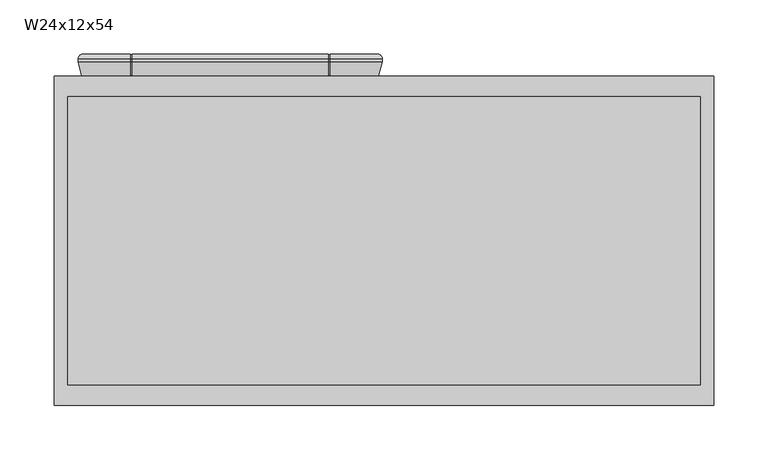
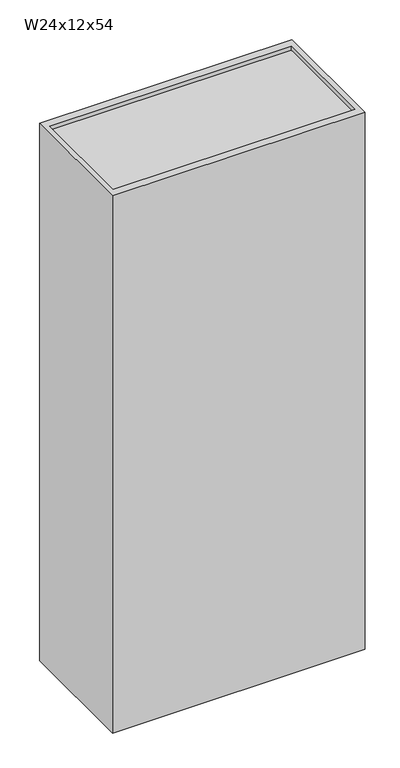
"""IFC4 building model written with IfcOpenShell, lengths in millimetres: furniture geometry, Cabinet-Wall-Merillat-Double_Door-Marlin : W24x12x54."""

from ifc_helpers import new_model, si_unit, frame, origin, place, context, project, spatial, polyline, circle_curve, ellipse_curve, outline, extrude, faceted_brep, source, transform, mapped, element, save
from ifc_brep_helpers import plane_surface, cylinder_surface, advanced_brep


def w24x12x54_3d81e8f6(model_context):
    return source(origin(), model_context, "Body", "SolidModel", [
        advanced_brep(
        [(-24.0971608, 382.5621, 2108.2), (-21.0006683, 387.0325, 2105.1035075), (-21.0006683, 387.0325, 790.4964925), (-24.0971608, 382.5621, 787.4), (-24.0971608, 379.7935, 787.4), (-24.0971608, 379.7935, 2108.2), (-20.5919608, 366.7125, 790.9052), (-20.5919608, 366.7125, 2104.6948), (24.104002, 366.7125, 2059.9988372), (24.104002, 366.7125, 835.6011628), (24.4741337, 367.50625, 835.9712945), (26.5552927, 371.96931, 838.0524535), (26.5552927, 371.96931, 2057.5475465), (24.4741337, 367.50625, 2059.6287055), (25.1555233, 374.2094093, 836.652684), (25.1555233, 374.2094093, 2058.947316), (10.8278392, 374.4595, 822.325), (10.8278392, 374.4595, 2073.275), (10.8278392, 379.2855, 822.325), (10.8278392, 379.2855, 2073.275), (25.1555233, 379.5355907, 836.652684), (25.1555233, 379.5355907, 2058.947316), (26.5552927, 381.77569, 838.0524535), (26.5552927, 381.77569, 2057.5475465), (24.4741337, 386.23875, 835.9712945), (24.1068694, 387.0263508, 835.6040302), (24.104002, 387.0325, 2059.9988372), (24.4741337, 386.23875, 2059.6287055), (24.1068694, 387.0325, 790.4964925), (24.1068694, 382.5621, 787.4), (253.7938467, 387.0325, 790.4964925), (256.8903392, 382.5621, 787.4), (208.7261206, 382.5621, 787.4), (208.7261206, 387.0325, 790.4964925), (25.6943694, 382.5621, 787.4), (25.6943694, 387.0325, 790.4964925), (207.1386206, 387.0325, 790.4964925), (207.1386206, 382.5621, 787.4), (24.1068694, 379.7935, 787.4), (256.8903392, 379.7935, 787.4), (208.7261206, 379.7935, 787.4), (25.6943694, 379.7935, 787.4), (207.1386206, 379.7935, 787.4), (24.1068694, 366.7125, 790.9052), (253.3851392, 366.7125, 790.9052), (208.7261206, 366.7125, 790.9052), (25.6943694, 366.7125, 790.9052), (207.1386206, 366.7125, 790.9052), (206.2378857, 371.96931, 838.0524535), (25.6943694, 367.50625, 835.9712945), (25.6943694, 366.7125, 835.6011628), (207.1386206, 366.7125, 835.6011628), (207.1386206, 367.50625, 835.9712945), (208.3190448, 367.50625, 835.9712945), (207.6376552, 374.2094093, 836.652684), (221.9653392, 374.4595, 822.325), (221.9653392, 379.2855, 822.325), (207.6376552, 379.5355907, 836.652684), (206.2378857, 381.77569, 838.0524535), (208.3190448, 386.23875, 835.9712945), (207.1386206, 386.23875, 835.9712945), (207.1386206, 387.0325, 835.6011628), (25.6943694, 387.0325, 835.6011628), (25.6943694, 386.23875, 835.9712945), (253.7938467, 387.0325, 2105.1035075), (256.8903392, 382.5621, 2108.2), (256.8903392, 379.7935, 2108.2), (253.3851392, 366.7125, 2104.6948), (208.6891765, 366.7125, 835.6011628), (208.6891765, 366.7125, 2059.9988372), (208.3190448, 367.50625, 2059.6287055), (206.2378857, 371.96931, 2057.5475465), (207.6376552, 374.2094093, 2058.947316), (221.9653392, 374.4595, 2073.275), (221.9653392, 379.2855, 2073.275), (207.6376552, 379.5355907, 2058.947316), (206.2378857, 381.77569, 2057.5475465), (208.3190448, 386.23875, 2059.6287055), (208.6891765, 387.0325, 2059.9988372), (208.6891765, 387.0325, 835.6011628), (208.7261206, 387.0325, 2105.1035075), (208.7261206, 382.5621, 2108.2), (24.1068694, 382.5621, 2108.2), (24.1068694, 387.0325, 2105.1035075), (207.1386206, 382.5621, 2108.2), (207.1386206, 387.0325, 2105.1035075), (25.6943694, 387.0325, 2105.1035075), (25.6943694, 382.5621, 2108.2), (208.7261206, 379.7935, 2108.2), (24.1068694, 379.7935, 2108.2), (207.1386206, 379.7935, 2108.2), (25.6943694, 379.7935, 2108.2), (208.7261206, 366.7125, 2104.6948), (24.1068694, 366.7125, 2104.6948), (207.1386206, 366.7125, 2104.6948), (25.6943694, 366.7125, 2104.6948), (207.1386206, 366.7125, 2059.9988372), (25.6943694, 366.7125, 2059.9988372), (207.1386206, 367.50625, 2059.6287055), (25.6943694, 367.50625, 2059.6287055), (25.6943694, 386.23875, 2059.6287055), (25.6943694, 387.0325, 2059.9988372), (207.1386206, 387.0325, 2059.9988372), (207.1386206, 386.23875, 2059.6287055), (207.1386206, 367.50625, 2104.0857412), (207.1386206, 379.8980037, 2107.40625), (207.1386206, 382.5621, 2107.40625), (207.1386206, 386.23875, 2104.9526052), (208.7261206, 386.23875, 2059.6287055), (208.7261206, 386.23875, 2104.9526052), (208.7261206, 382.5621, 2107.40625), (208.7261206, 379.8980037, 2107.40625), (208.7261206, 367.50625, 2104.0857412), (208.7261206, 367.50625, 2059.6287055), (24.1068694, 367.50625, 2059.6287055), (24.1068694, 367.50625, 2104.0857412), (24.1068694, 379.8980037, 2107.40625), (24.1068694, 382.5621, 2107.40625), (24.1068694, 386.23875, 2104.9526052), (24.1068694, 386.23875, 2059.6287055), (25.6943694, 386.23875, 2104.9526052), (25.6943694, 382.5621, 2107.40625), (25.6943694, 379.8980037, 2107.40625), (25.6943694, 367.50625, 2104.0857412), (24.1068694, 386.23875, 835.9712945), (24.1068694, 386.23875, 790.6473948), (24.1068694, 382.5621, 788.19375), (24.1068694, 379.8980037, 788.19375), (24.1068694, 367.50625, 791.5142588), (24.1068694, 367.50625, 835.9712945), (25.6943694, 367.50625, 791.5142588), (25.6943694, 379.8980037, 788.19375), (25.6943694, 382.5621, 788.19375), (25.6943694, 386.23875, 790.6473948), (207.1386206, 386.23875, 790.6473948), (207.1386206, 382.5621, 788.19375), (207.1386206, 379.8980037, 788.19375), (207.1386206, 367.50625, 791.5142588), (208.7261206, 386.23875, 835.9712945), (208.7261206, 367.50625, 835.9712945), (208.7261206, 367.50625, 791.5142588), (208.7261206, 379.8980037, 788.19375), (208.7261206, 382.5621, 788.19375), (208.7261206, 386.23875, 790.6473948)],
        [
            (0, 1, ellipse_curve(frame((-19.3219608, 382.5621, 2103.4248), z_axis=(-0.7071067811865475, 0.0, -0.7071067811865475), x_axis=(-0.7071067811865474, 0.0, 0.7071067811865476)), 6.7531526, 4.7752)),
            (1, 2),
            (2, 3, ellipse_curve(frame((-19.3219608, 382.5621, 792.1752), z_axis=(-0.7071067811865475, 0.0, 0.7071067811865475), x_axis=(0.7071067811865474, 0.0, 0.7071067811865476)), 6.7531526, 4.7752)),
            (3, 0),
            (3, 4),
            (4, 5),
            (5, 0),
            (4, 6),
            (6, 7),
            (7, 5),
            (8, 9),
            (9, 10),
            (10, 11),
            (11, 12),
            (12, 13),
            (13, 8),
            (11, 14, ellipse_curve(frame((25.1280392, 372.6348492, 836.6252), z_axis=(-0.7071067811865475, 0.0, 0.7071067811865475), x_axis=(0.7071067811865474, 0.0, 0.7071067811865476)), 2.2271035, 1.5748)),
            (14, 15),
            (15, 12, ellipse_curve(frame((25.1280392, 372.6348492, 2058.9748), z_axis=(-0.7071067811865475, 0.0, -0.7071067811865475), x_axis=(-0.7071067811865474, 0.0, 0.7071067811865476)), 2.2271035, 1.5748)),
            (14, 16),
            (16, 17),
            (17, 15),
            (16, 18),
            (18, 19),
            (19, 17),
            (18, 20),
            (20, 21),
            (21, 19),
            (20, 22, ellipse_curve(frame((25.1280392, 381.1101508, 836.6252), z_axis=(-0.7071067811865475, 0.0, 0.7071067811865475), x_axis=(0.7071067811865474, 0.0, 0.7071067811865476)), 2.2271035, 1.5748)),
            (22, 23),
            (23, 21, ellipse_curve(frame((25.1280392, 381.1101508, 2058.9748), z_axis=(-0.7071067811865475, 0.0, -0.7071067811865475), x_axis=(-0.7071067811865474, 0.0, 0.7071067811865476)), 2.2271035, 1.5748)),
            (22, 24),
            (24, 25),
            (25, 26),
            (26, 27),
            (27, 23),
            (2, 28),
            (28, 29, circle_curve(frame((24.1068694, 382.5621, 792.1752), z_axis=(-1.0, 0.0, 0.0), x_axis=(0.0, -1.0, 0.0)), 4.7752)),
            (29, 3),
            (30, 31, ellipse_curve(frame((252.1151392, 382.5621, 792.1752), z_axis=(-0.7071067811865475, 0.0, -0.7071067811865475), x_axis=(-0.7071067811865476, 0.0, 0.7071067811865474)), 6.7531526, 4.7752)),
            (31, 32),
            (32, 33, circle_curve(frame((208.7261206, 382.5621, 792.1752), z_axis=(1.0, 0.0, 0.0), x_axis=(0.0, -1.0, 0.0)), 4.7752)),
            (33, 30),
            (34, 35, circle_curve(frame((25.6943694, 382.5621, 792.1752), z_axis=(1.0, 0.0, 0.0), x_axis=(0.0, -1.0, 0.0)), 4.7752)),
            (35, 36),
            (36, 37, circle_curve(frame((207.1386206, 382.5621, 792.1752), z_axis=(-1.0, 0.0, 0.0), x_axis=(0.0, -1.0, 0.0)), 4.7752)),
            (37, 34),
            (29, 38),
            (38, 4),
            (31, 39),
            (39, 40),
            (40, 32),
            (41, 34),
            (37, 42),
            (42, 41),
            (38, 43),
            (43, 6),
            (39, 44),
            (44, 45),
            (45, 40),
            (46, 41),
            (42, 47),
            (47, 46),
            (48, 11),
            (10, 49),
            (49, 50),
            (50, 51),
            (51, 52),
            (52, 53),
            (53, 48),
            (48, 54, ellipse_curve(frame((207.6651392, 372.6348492, 836.6252), z_axis=(-0.7071067811865475, 0.0, -0.7071067811865475), x_axis=(-0.7071067811865476, 0.0, 0.7071067811865474)), 2.2271035, 1.5748)),
            (54, 14),
            (54, 55),
            (55, 16),
            (55, 56),
            (56, 18),
            (56, 57),
            (57, 20),
            (57, 58, ellipse_curve(frame((207.6651392, 381.1101508, 836.6252), z_axis=(-0.7071067811865475, 0.0, -0.7071067811865475), x_axis=(-0.7071067811865476, 0.0, 0.7071067811865474)), 2.2271035, 1.5748)),
            (58, 22),
            (58, 59),
            (59, 60),
            (60, 61),
            (61, 62),
            (62, 63),
            (63, 24),
            (30, 64),
            (64, 65, ellipse_curve(frame((252.1151392, 382.5621, 2103.4248), z_axis=(0.7071067811865475, 0.0, -0.7071067811865475), x_axis=(-0.7071067811865474, 0.0, -0.7071067811865476)), 6.7531526, 4.7752)),
            (65, 31),
            (65, 66),
            (66, 39),
            (66, 67),
            (67, 44),
            (68, 69),
            (69, 70),
            (70, 71),
            (71, 48),
            (53, 68),
            (71, 72, ellipse_curve(frame((207.6651392, 372.6348492, 2058.9748), z_axis=(0.7071067811865475, 0.0, -0.7071067811865475), x_axis=(-0.7071067811865474, 0.0, -0.7071067811865476)), 2.2271035, 1.5748)),
            (72, 54),
            (72, 73),
            (73, 55),
            (73, 74),
            (74, 56),
            (74, 75),
            (75, 57),
            (75, 76, ellipse_curve(frame((207.6651392, 381.1101508, 2058.9748), z_axis=(0.7071067811865475, 0.0, -0.7071067811865475), x_axis=(-0.7071067811865474, 0.0, -0.7071067811865476)), 2.2271035, 1.5748)),
            (76, 58),
            (76, 77),
            (77, 78),
            (78, 79),
            (79, 59),
            (64, 80),
            (80, 81, circle_curve(frame((208.7261206, 382.5621, 2103.4248), z_axis=(1.0, 0.0, 0.0), x_axis=(0.0, -1.0, 0.0)), 4.7752)),
            (81, 65),
            (0, 82),
            (82, 83, circle_curve(frame((24.1068694, 382.5621, 2103.4248), z_axis=(-1.0, 0.0, 0.0), x_axis=(0.0, -1.0, 0.0)), 4.7752)),
            (83, 1),
            (84, 85, circle_curve(frame((207.1386206, 382.5621, 2103.4248), z_axis=(-1.0, 0.0, 0.0), x_axis=(0.0, -1.0, 0.0)), 4.7752)),
            (85, 86),
            (86, 87, circle_curve(frame((25.6943694, 382.5621, 2103.4248), z_axis=(1.0, 0.0, 0.0), x_axis=(0.0, -1.0, 0.0)), 4.7752)),
            (87, 84),
            (81, 88),
            (88, 66),
            (5, 89),
            (89, 82),
            (90, 84),
            (87, 91),
            (91, 90),
            (88, 92),
            (92, 67),
            (7, 93),
            (93, 89),
            (94, 90),
            (91, 95),
            (95, 94),
            (43, 9),
            (8, 93),
            (92, 69),
            (68, 45),
            (96, 94),
            (95, 97),
            (97, 96),
            (50, 46),
            (47, 51),
            (12, 71),
            (70, 98),
            (98, 96),
            (97, 99),
            (99, 13),
            (15, 72),
            (17, 73),
            (19, 74),
            (21, 75),
            (23, 76),
            (27, 100),
            (100, 101),
            (101, 102),
            (102, 103),
            (103, 77),
            (83, 26),
            (25, 28),
            (33, 79),
            (78, 80),
            (85, 102),
            (101, 86),
            (35, 62),
            (61, 36),
            (98, 104),
            (104, 105),
            (105, 106),
            (106, 107, circle_curve(frame((207.1386206, 382.5621, 2103.4248), z_axis=(-1.0, 0.0, 0.0), x_axis=(0.0, 0.0, 1.0)), 3.98145)),
            (107, 103),
            (78, 108),
            (108, 109),
            (109, 110, circle_curve(frame((208.7261206, 382.5621, 2103.4248), z_axis=(1.0, 0.0, 0.0), x_axis=(0.0, 0.0, 1.0)), 3.98145)),
            (110, 111),
            (111, 112),
            (112, 113),
            (113, 69),
            (77, 108),
            (107, 109),
            (106, 110),
            (105, 111),
            (104, 112),
            (70, 113),
            (8, 114),
            (114, 115),
            (115, 116),
            (116, 117),
            (117, 118, circle_curve(frame((24.1068694, 382.5621, 2103.4248), z_axis=(-1.0, 0.0, 0.0), x_axis=(0.0, 0.0, 1.0)), 3.98145)),
            (118, 119),
            (119, 26),
            (100, 120),
            (120, 121, circle_curve(frame((25.6943694, 382.5621, 2103.4248), z_axis=(1.0, 0.0, 0.0), x_axis=(0.0, 0.0, 1.0)), 3.98145)),
            (121, 122),
            (122, 123),
            (123, 99),
            (119, 27),
            (118, 120),
            (117, 121),
            (116, 122),
            (115, 123),
            (114, 13),
            (25, 124),
            (124, 125),
            (125, 126, circle_curve(frame((24.1068694, 382.5621, 792.1752), z_axis=(-1.0, 0.0, 0.0), x_axis=(0.0, 0.0, 1.0)), 3.98145)),
            (126, 127),
            (127, 128),
            (128, 129),
            (129, 9),
            (49, 130),
            (130, 131),
            (131, 132),
            (132, 133, circle_curve(frame((25.6943694, 382.5621, 792.1752), z_axis=(1.0, 0.0, 0.0), x_axis=(0.0, 0.0, 1.0)), 3.98145)),
            (133, 63),
            (129, 10),
            (128, 130),
            (127, 131),
            (126, 132),
            (125, 133),
            (124, 24),
            (60, 134),
            (134, 135, circle_curve(frame((207.1386206, 382.5621, 792.1752), z_axis=(-1.0, 0.0, 0.0), x_axis=(0.0, 0.0, 1.0)), 3.98145)),
            (135, 136),
            (136, 137),
            (137, 52),
            (138, 79),
            (68, 139),
            (139, 140),
            (140, 141),
            (141, 142),
            (142, 143, circle_curve(frame((208.7261206, 382.5621, 792.1752), z_axis=(1.0, 0.0, 0.0), x_axis=(0.0, 0.0, 1.0)), 3.98145)),
            (143, 138),
            (138, 59),
            (53, 139),
            (137, 140),
            (136, 141),
            (135, 142),
            (134, 143),
        ],
        [
            cylinder_surface(frame((-19.3219608, 382.5621, 2108.2), z_axis=(0.0, 0.0, 1.0), x_axis=(0.0, -1.0, 0.0)), 4.7752),
            plane_surface(frame((-24.0971608, 382.5621, 2108.2), z_axis=(-1.0, 0.0, 0.0), x_axis=(0.0, 0.0, -1.0))),
            plane_surface(frame((-24.0971608, 379.7935, 2108.2), z_axis=(-0.9659229350723619, -0.25882983502910506, 0.0), x_axis=(0.0, 0.0, -1.0))),
            plane_surface(frame((24.104002, 366.7125, 2059.9988372), z_axis=(0.9063077870366099, -0.4226182617407856, 0.0), x_axis=(0.0, 0.0, -1.0))),
            cylinder_surface(frame((25.1280392, 372.6348492, 2108.2), z_axis=(0.0, 0.0, 1.0000000000000002), x_axis=(0.01745240643729364, 0.9998476951563912, 0.0)), 1.5748),
            plane_surface(frame((25.1555233, 374.2094093, 2058.947316), z_axis=(0.017452406437322144, 0.9998476951563906, 0.0), x_axis=(0.0, 0.0, -1.0))),
            plane_surface(frame((10.8278392, 374.4595, 2073.275), z_axis=(1.0, 0.0, 0.0), x_axis=(0.0, 0.0, -1.0))),
            plane_surface(frame((10.8278392, 379.2855, 2073.275), z_axis=(0.01745240643727848, -0.9998476951563914, 0.0), x_axis=(0.0, 0.0, -1.0))),
            cylinder_surface(frame((25.1280392, 381.1101508, 2108.2), z_axis=(0.0, 0.0, 1.0000000000000002), x_axis=(0.9063077870367326, 0.42261826174052236, 0.0)), 1.5748),
            plane_surface(frame((26.5552927, 381.77569, 2057.5475465), z_axis=(0.9063077870366333, 0.4226182617407352, 0.0), x_axis=(0.0, 0.0, -1.0))),
            cylinder_surface(frame((-24.0971608, 382.5621, 792.1752), z_axis=(-1.0, 0.0, 0.0), x_axis=(0.0, -1.0, 0.0)), 4.7752),
            plane_surface(frame((-24.0971608, 382.5621, 787.4), z_axis=(0.0, 0.0, -1.0), x_axis=(1.0, 0.0, 0.0))),
            plane_surface(frame((-24.0971608, 379.7935, 787.4), z_axis=(0.0, -0.2588298350291095, -0.9659229350723607), x_axis=(1.0, 0.0, 0.0))),
            plane_surface(frame((24.104002, 366.7125, 835.6011628), z_axis=(0.0, -0.42261826174078143, 0.9063077870366119), x_axis=(1.0, 0.0, 0.0))),
            cylinder_surface(frame((-24.0971608, 372.6348492, 836.6252), z_axis=(-1.0000000000000002, 0.0, 0.0), x_axis=(0.0, 0.9998476951563913, 0.017452406437289025)), 1.5748),
            plane_surface(frame((25.1555233, 374.2094093, 836.652684), z_axis=(0.0, 0.9998476951563907, 0.01745240643731753), x_axis=(1.0, 0.0, 0.0))),
            plane_surface(frame((10.8278392, 374.4595, 822.325), z_axis=(0.0, 0.0, 1.0), x_axis=(1.0, 0.0, 0.0))),
            plane_surface(frame((10.8278392, 379.2855, 822.325), z_axis=(0.0, -0.9998476951563913, 0.017452406437283095), x_axis=(1.0, 0.0, 0.0))),
            cylinder_surface(frame((-24.0971608, 381.1101508, 836.6252), z_axis=(-1.0000000000000002, 0.0, 0.0), x_axis=(0.0, 0.4226182617405265, 0.9063077870367306)), 1.5748),
            plane_surface(frame((26.5552927, 381.77569, 838.0524535), z_axis=(0.0, 0.4226182617407394, 0.9063077870366314), x_axis=(1.0, 0.0, 0.0))),
            cylinder_surface(frame((252.1151392, 382.5621, 787.4), z_axis=(0.0, 0.0, -1.0), x_axis=(0.0, -1.0, 0.0)), 4.7752),
            plane_surface(frame((256.8903392, 382.5621, 787.4), z_axis=(1.0, 0.0, 0.0), x_axis=(0.0, 0.0, 1.0))),
            plane_surface(frame((256.8903392, 379.7935, 787.4), z_axis=(0.9659229350723619, -0.25882983502910506, 0.0), x_axis=(0.0, 0.0, 1.0))),
            plane_surface(frame((208.6891765, 366.7125, 835.6011628), z_axis=(-0.9063077870366099, -0.4226182617407856, 0.0), x_axis=(0.0, 0.0, 1.0))),
            cylinder_surface(frame((207.6651392, 372.6348492, 787.4), z_axis=(0.0, 0.0, -1.0000000000000002), x_axis=(-0.01745240643729364, 0.9998476951563912, 0.0)), 1.5748),
            plane_surface(frame((207.6376552, 374.2094093, 836.652684), z_axis=(-0.017452406437322144, 0.9998476951563906, 0.0), x_axis=(0.0, 0.0, 1.0))),
            plane_surface(frame((221.9653392, 374.4595, 822.325), z_axis=(-1.0, 0.0, 0.0), x_axis=(0.0, 0.0, 1.0))),
            plane_surface(frame((221.9653392, 379.2855, 822.325), z_axis=(-0.01745240643727848, -0.9998476951563914, 0.0), x_axis=(0.0, 0.0, 1.0))),
            cylinder_surface(frame((207.6651392, 381.1101508, 787.4), z_axis=(0.0, 0.0, -1.0000000000000002), x_axis=(-0.9063077870367326, 0.42261826174052236, 0.0)), 1.5748),
            plane_surface(frame((206.2378857, 381.77569, 838.0524535), z_axis=(-0.9063077870366333, 0.4226182617407352, 0.0), x_axis=(0.0, 0.0, 1.0))),
            cylinder_surface(frame((256.8903392, 382.5621, 2103.4248), z_axis=(1.0, 0.0, 0.0), x_axis=(0.0, -1.0, 0.0)), 4.7752),
            plane_surface(frame((256.8903392, 382.5621, 2108.2), z_axis=(0.0, 0.0, 1.0), x_axis=(-1.0, 0.0, 0.0))),
            plane_surface(frame((256.8903392, 379.7935, 2108.2), z_axis=(0.0, -0.2588298350291006, 0.9659229350723632), x_axis=(-1.0, 0.0, 0.0))),
            plane_surface(frame((253.3851392, 366.7125, 2104.6948), z_axis=(0.0, -1.0, 0.0), x_axis=(-1.0, 0.0, 0.0))),
            plane_surface(frame((208.6891765, 366.7125, 2059.9988372), z_axis=(0.0, -0.42261826174078976, -0.9063077870366079), x_axis=(-1.0, 0.0, 0.0))),
            cylinder_surface(frame((256.8903392, 372.6348492, 2058.9748), z_axis=(1.0000000000000002, 0.0, 0.0), x_axis=(0.0, 0.999847695156391, -0.017452406437298253)), 1.5748),
            plane_surface(frame((207.6376552, 374.2094093, 2058.947316), z_axis=(0.0, 0.9998476951563905, -0.01745240643732676), x_axis=(-1.0, 0.0, 0.0))),
            plane_surface(frame((221.9653392, 374.4595, 2073.275), z_axis=(0.0, 0.0, -1.0), x_axis=(-1.0, 0.0, 0.0))),
            plane_surface(frame((221.9653392, 379.2855, 2073.275), z_axis=(0.0, -0.9998476951563915, -0.017452406437273867), x_axis=(-1.0, 0.0, 0.0))),
            cylinder_surface(frame((256.8903392, 381.1101508, 2058.9748), z_axis=(1.0000000000000002, 0.0, 0.0), x_axis=(0.0, 0.4226182617405182, -0.9063077870367346)), 1.5748),
            plane_surface(frame((206.2378857, 381.77569, 2057.5475465), z_axis=(0.0, 0.422618261740731, -0.9063077870366353), x_axis=(-1.0, 0.0, 0.0))),
            plane_surface(frame((208.6891765, 387.0325, 2059.9988372), z_axis=(0.0, 1.0, 0.0), x_axis=(-1.0, 0.0, 0.0))),
            plane_surface(frame((207.1386206, 387.0325, 2059.9988372), z_axis=(1.0000000000000002, 0.0, 0.0), x_axis=(0.0, -0.9063077870366177, -0.4226182617407689))),
            plane_surface(frame((208.7261206, 387.0325, 2059.9988372), z_axis=(-1.0000000000000002, 0.0, 0.0), x_axis=(0.0, 0.9063077870366177, 0.4226182617407689))),
            plane_surface(frame((207.1386206, 387.0325, 2059.9988372), z_axis=(0.0, -0.4226182617407689, 0.9063077870366177), x_axis=(1.0, 0.0, 0.0))),
            plane_surface(frame((207.1386206, 386.23875, 2059.6287055), z_axis=(0.0, 1.0, 0.0), x_axis=(1.0, 0.0, 0.0))),
            cylinder_surface(frame((208.7261206, 382.5621, 2103.4248), z_axis=(1.0, 0.0, 0.0), x_axis=(0.0, 0.0, 1.0)), 3.98145),
            plane_surface(frame((207.1386206, 382.5621, 2107.40625), z_axis=(0.0, 0.0, 1.0), x_axis=(1.0, 0.0, 0.0))),
            plane_surface(frame((207.1386206, 379.8980037, 2107.40625), z_axis=(0.0, -0.2588298350291571, 0.965922935072348), x_axis=(1.0, 0.0, 0.0))),
            plane_surface(frame((207.1386206, 367.50625, 2104.0857412), z_axis=(0.0, -1.0, 0.0), x_axis=(1.0, 0.0, 0.0))),
            plane_surface(frame((207.1386206, 367.50625, 2059.6287055), z_axis=(0.0, 0.4226182617408151, 0.906307787036596), x_axis=(1.0, 0.0, 0.0))),
            plane_surface(frame((24.1068694, 387.0325, 2059.9988372), z_axis=(1.0, 0.0, 0.0), x_axis=(0.0, -0.9063077870366254, -0.42261826174075223))),
            plane_surface(frame((25.6943694, 387.0325, 2059.9988372), z_axis=(-1.0, 0.0, 0.0), x_axis=(0.0, 0.9063077870366254, 0.42261826174075223))),
            plane_surface(frame((24.1068694, 387.0325, 2059.9988372), z_axis=(0.0, -0.42261826174075223, 0.9063077870366254), x_axis=(1.0, 0.0, 0.0))),
            plane_surface(frame((24.1068694, 386.23875, 2059.6287055), z_axis=(0.0, 1.0, 0.0), x_axis=(1.0, 0.0, 0.0))),
            cylinder_surface(frame((25.6943694, 382.5621, 2103.4248), z_axis=(1.0, 0.0, 0.0), x_axis=(0.0, 0.0, 1.0)), 3.98145),
            plane_surface(frame((24.1068694, 382.5621, 2107.40625), z_axis=(0.0, 0.0, 1.0), x_axis=(1.0, 0.0, 0.0))),
            plane_surface(frame((24.1068694, 379.8980037, 2107.40625), z_axis=(0.0, -0.258829835029159, 0.9659229350723475), x_axis=(1.0, 0.0, 0.0))),
            plane_surface(frame((24.1068694, 367.50625, 2104.0857412), z_axis=(0.0, -1.0, 0.0), x_axis=(1.0, 0.0, 0.0))),
            plane_surface(frame((24.1068694, 367.50625, 2059.6287055), z_axis=(0.0, 0.4226182617408322, 0.9063077870365881), x_axis=(1.0, 0.0, 0.0))),
            plane_surface(frame((24.1068694, 382.5621, 796.9504), z_axis=(1.0, 0.0, 0.0), x_axis=(0.0, 1.0, 0.0))),
            plane_surface(frame((25.6943694, 382.5621, 796.9504), z_axis=(-1.0, 0.0, 0.0), x_axis=(0.0, -1.0, 0.0))),
            plane_surface(frame((24.1068694, 366.7125, 835.6011628), z_axis=(0.0, 0.4226182617407559, -0.9063077870366237), x_axis=(1.0, 0.0, 0.0))),
            plane_surface(frame((24.1068694, 367.50625, 835.9712945), z_axis=(0.0, -1.0, 0.0), x_axis=(1.0, 0.0, 0.0))),
            plane_surface(frame((24.1068694, 367.50625, 791.5142588), z_axis=(0.0, -0.25882983502944146, -0.9659229350722718), x_axis=(1.0, 0.0, 0.0))),
            plane_surface(frame((24.1068694, 379.8980037, 788.19375), z_axis=(0.0, 0.0, -1.0), x_axis=(1.0, 0.0, 0.0))),
            cylinder_surface(frame((25.6943694, 382.5621, 792.1752), z_axis=(1.0, 0.0, 0.0), x_axis=(0.0, 0.0, 1.0)), 3.98145),
            plane_surface(frame((24.1068694, 386.23875, 790.6473948), z_axis=(0.0, 1.0, 0.0), x_axis=(1.0, 0.0, 0.0))),
            plane_surface(frame((24.1068694, 386.23875, 835.9712945), z_axis=(0.0, -0.42261826174073325, -0.9063077870366342), x_axis=(1.0, 0.0, 0.0))),
            plane_surface(frame((207.1386206, 386.23875, 835.9712945), z_axis=(1.0, 0.0, 0.0), x_axis=(0.0, 0.9063077870366539, -0.42261826174069095))),
            plane_surface(frame((208.7261206, 386.23875, 835.9712945), z_axis=(-1.0, 0.0, 0.0), x_axis=(0.0, -0.9063077870366539, 0.42261826174069095))),
            plane_surface(frame((207.1386206, 386.23875, 835.9712945), z_axis=(0.0, -0.42261826174069095, -0.9063077870366539), x_axis=(1.0, 0.0, 0.0))),
            plane_surface(frame((207.1386206, 366.7125, 835.6011628), z_axis=(0.0, 0.42261826174079387, -0.9063077870366061), x_axis=(1.0, 0.0, 0.0))),
            plane_surface(frame((207.1386206, 367.50625, 835.9712945), z_axis=(0.0, -1.0, 0.0), x_axis=(1.0, 0.0, 0.0))),
            plane_surface(frame((207.1386206, 367.50625, 791.5142588), z_axis=(0.0, -0.25882983502944, -0.9659229350722722), x_axis=(1.0, 0.0, 0.0))),
            plane_surface(frame((207.1386206, 379.8980037, 788.19375), z_axis=(0.0, 0.0, -1.0), x_axis=(1.0, 0.0, 0.0))),
            cylinder_surface(frame((208.7261206, 382.5621, 792.1752), z_axis=(1.0, 0.0, 0.0), x_axis=(0.0, 0.0, 1.0)), 3.98145),
            plane_surface(frame((207.1386206, 386.23875, 790.6473948), z_axis=(0.0, 1.0, 0.0), x_axis=(1.0, 0.0, 0.0))),
        ],
        [
            (0, [[1, 2, 3, 4]]),
            (1, [[-4, 5, 6, 7]]),
            (2, [[-6, 8, 9, 10]]),
            (3, [[11, 12, 13, 14, 15, 16]]),
            (4, [[-14, 17, 18, 19]]),
            (5, [[-18, 20, 21, 22]]),
            (6, [[-21, 23, 24, 25]]),
            (7, [[-24, 26, 27, 28]]),
            (8, [[-27, 29, 30, 31]]),
            (9, [[-30, 32, 33, 34, 35, 36]]),
            (10, [[-3, 37, 38, 39]]),
            (10, [[40, 41, 42, 43]]),
            (10, [[44, 45, 46, 47]]),
            (11, [[-5, -39, 48, 49]]),
            (11, [[50, 51, 52, -41]]),
            (11, [[53, -47, 54, 55]]),
            (12, [[-8, -49, 56, 57]]),
            (12, [[58, 59, 60, -51]]),
            (12, [[61, -55, 62, 63]]),
            (13, [[64, -13, 65, 66, 67, 68, 69, 70]]),
            (14, [[-17, -64, 71, 72]]),
            (15, [[-20, -72, 73, 74]]),
            (16, [[-23, -74, 75, 76]]),
            (17, [[-26, -76, 77, 78]]),
            (18, [[-29, -78, 79, 80]]),
            (19, [[-80, 81, 82, 83, 84, 85, 86, -32]]),
            (20, [[-40, 87, 88, 89]]),
            (21, [[-50, -89, 90, 91]]),
            (22, [[-58, -91, 92, 93]]),
            (23, [[94, 95, 96, 97, -70, 98]]),
            (24, [[-71, -97, 99, 100]]),
            (25, [[-73, -100, 101, 102]]),
            (26, [[-75, -102, 103, 104]]),
            (27, [[-77, -104, 105, 106]]),
            (28, [[-79, -106, 107, 108]]),
            (29, [[-108, 109, 110, 111, 112, -81]]),
            (30, [[-88, 113, 114, 115]]),
            (30, [[-1, 116, 117, 118]]),
            (30, [[119, 120, 121, 122]]),
            (31, [[-90, -115, 123, 124]]),
            (31, [[-7, 125, 126, -116]]),
            (31, [[127, -122, 128, 129]]),
            (32, [[-92, -124, 130, 131]]),
            (32, [[-10, 132, 133, -125]]),
            (32, [[134, -129, 135, 136]]),
            (33, [[-9, -57, 137, -11, 138, -132]]),
            (33, [[-93, -131, 139, -94, 140, -59]]),
            (33, [[141, -136, 142, 143]]),
            (33, [[144, -63, 145, -67]]),
            (34, [[146, -96, 147, 148, -143, 149, 150, -15]]),
            (35, [[-19, 151, -99, -146]]),
            (36, [[-22, 152, -101, -151]]),
            (37, [[-25, 153, -103, -152]]),
            (38, [[-28, 154, -105, -153]]),
            (39, [[-31, 155, -107, -154]]),
            (40, [[-155, -36, 156, 157, 158, 159, 160, -109]]),
            (41, [[-2, -118, 161, -34, 162, -37]]),
            (41, [[-87, -43, 163, -111, 164, -113]]),
            (41, [[165, -158, 166, -120]]),
            (41, [[167, -84, 168, -45]]),
            (42, [[169, 170, 171, 172, 173, -159, -165, -119, -127, -134, -141, -148]]),
            (43, [[174, 175, 176, 177, 178, 179, 180, -139, -130, -123, -114, -164]]),
            (44, [[-174, -110, 181]]),
            (45, [[-173, 182, -175, -181, -160]]),
            (46, [[-172, 183, -176, -182]]),
            (47, [[-171, 184, -177, -183]]),
            (48, [[-170, 185, -178, -184]]),
            (49, [[-169, -147, 186, -179, -185]]),
            (50, [[-180, -186, -95]]),
            (51, [[187, 188, 189, 190, 191, 192, 193, -161, -117, -126, -133, -138]]),
            (52, [[194, 195, 196, 197, 198, -149, -142, -135, -128, -121, -166, -157]]),
            (53, [[-193, 199, -35]]),
            (54, [[-192, 200, -194, -156, -199]]),
            (55, [[-191, 201, -195, -200]]),
            (56, [[-190, 202, -196, -201]]),
            (57, [[-189, 203, -197, -202]]),
            (58, [[-188, 204, -150, -198, -203]]),
            (59, [[-187, -16, -204]]),
            (60, [[205, 206, 207, 208, 209, 210, 211, -137, -56, -48, -38, -162]]),
            (61, [[212, 213, 214, 215, 216, -85, -167, -44, -53, -61, -144, -66]]),
            (62, [[-211, 217, -12]]),
            (63, [[-210, 218, -212, -65, -217]]),
            (64, [[-209, 219, -213, -218]]),
            (65, [[-208, 220, -214, -219]]),
            (66, [[-207, 221, -215, -220]]),
            (67, [[-206, 222, -86, -216, -221]]),
            (68, [[-205, -33, -222]]),
            (69, [[223, 224, 225, 226, 227, -68, -145, -62, -54, -46, -168, -83]]),
            (70, [[228, -163, -42, -52, -60, -140, 229, 230, 231, 232, 233, 234]]),
            (71, [[-228, 235, -112]]),
            (72, [[-229, -98, 236]]),
            (73, [[-227, 237, -230, -236, -69]]),
            (74, [[-226, 238, -231, -237]]),
            (75, [[-225, 239, -232, -238]]),
            (76, [[-224, 240, -233, -239]]),
            (77, [[-223, -82, -235, -234, -240]]),
        ],
    ),
        extrude(outline(polyline([(221.9653392, 379.2855), (221.9653392, 374.4595), (10.8278392, 374.4595), (10.8278392, 379.2855), (221.9653392, 379.2855)])), frame((0.0, 0.0, 822.325), z_axis=(0.0, 0.0, 1.0), x_axis=(1.0, 0.0, 0.0)), (0.0, 0.0, 1.0), 1250.95),
        extrude(outline(polyline([(-8.5711577, 347.6625), (525.0128185, 347.6625), (525.0128185, 80.9625), (-8.5711577, 80.9625), (-8.5711577, 347.6625)])), frame((0.0, 0.0, 1800.225), z_axis=(0.0, 0.0, 1.0), x_axis=(1.0, 0.0, 0.0)), (0.0, 0.0, 1.0), 19.05),
        extrude(outline(polyline([(-8.5711577, 347.6625), (525.0128185, 347.6625), (525.0128185, 80.9625), (-8.5711577, 80.9625), (-8.5711577, 347.6625)])), frame((0.0, 0.0, 1076.325), z_axis=(0.0, 0.0, 1.0), x_axis=(1.0, 0.0, 0.0)), (0.0, 0.0, 1.0), 19.05),
        extrude(outline(polyline([(-8.5711577, 347.6625), (525.0128185, 347.6625), (525.0128185, 80.9625), (-8.5711577, 80.9625), (-8.5711577, 347.6625)])), frame((0.0, 0.0, 1438.275), z_axis=(0.0, 0.0, 1.0), x_axis=(1.0, 0.0, 0.0)), (0.0, 0.0, 1.0), 19.05),
        faceted_brep([(-46.3221608, 61.9125, 2133.6), (-46.3221608, 61.9125, 762.0), (563.2778392, 61.9125, 762.0), (563.2778392, 61.9125, 2133.6), (-46.3221608, 366.7125, 2133.6), (563.2778392, 366.7125, 2133.6), (563.2778392, 366.7125, 762.0), (-46.3221608, 366.7125, 762.0), (525.0128185, 366.7125, 2095.2735163), (301.9690685, 366.7125, 2095.2735163), (301.9690685, 366.7125, 799.8672696), (525.0128185, 366.7125, 799.8672696), (-8.5711577, 366.7125, 2095.2735163), (-8.5711577, 366.7125, 799.8672696), (214.98661, 366.7125, 799.8672696), (214.98661, 366.7125, 2095.2735163), (-33.6221608, 80.9625, 762.0), (550.5778392, 80.9625, 762.0), (550.5778392, 347.6625, 762.0), (-33.6221608, 347.6625, 762.0), (550.5778392, 347.6625, 2133.6), (550.5778392, 80.9625, 2133.6), (-33.6221608, 80.9625, 2133.6), (-33.6221608, 347.6625, 2133.6), (-8.5711577, 80.9625, 2095.2735163), (214.98661, 347.6625, 2095.2735163), (301.9690685, 347.6625, 2095.2735163), (525.0128185, 80.9625, 2095.2735163), (525.0128185, 80.9625, 799.8672696), (301.9690685, 347.6625, 799.8672696), (214.98661, 347.6625, 799.8672696), (-8.5711577, 80.9625, 799.8672696), (550.5778392, 80.9625, 2122.9851371), (550.5778392, 347.6625, 2122.9851371), (-33.6221608, 347.6625, 2122.9851371), (-33.6221608, 80.9625, 2122.9851371), (-33.6221608, 80.9625, 771.8352657), (-33.6221608, 347.6625, 771.8352657), (550.5778392, 347.6625, 771.8352657), (550.5778392, 80.9625, 771.8352657)], [[[0, 1, 2, 3]], [[4, 5, 6, 7], [8, 9, 10, 11], [12, 13, 14, 15]], [[1, 0, 4, 7]], [[2, 1, 7, 6], [16, 17, 18, 19]], [[3, 2, 6, 5]], [[0, 3, 5, 4], [20, 21, 22, 23]], [[24, 12, 15, 25, 26, 9, 8, 27]], [[8, 11, 28, 27]], [[28, 11, 10, 29, 30, 14, 13, 31]], [[13, 12, 24, 31]], [[32, 33, 34, 35]], [[33, 32, 21, 20]], [[34, 33, 20, 23]], [[35, 34, 23, 22]], [[32, 35, 22, 21]], [[36, 37, 38, 39]], [[36, 39, 17, 16]], [[39, 38, 18, 17]], [[38, 37, 19, 18]], [[37, 36, 16, 19]], [[24, 27, 28, 31]], [[26, 29, 10, 9]], [[15, 14, 30, 25]], [[29, 26, 25, 30]]]),
    ])


if __name__ == "__main__":
    model = new_model("IFC4")
    model_context = context("Model", 3, world=origin())
    ifc_project = project(units=[si_unit("LENGTHUNIT", "METRE", prefix="MILLI")], contexts=[model_context])
    site = spatial("IfcSite", under=ifc_project)
    building = spatial("IfcBuilding", under=site)
    placement = place(None, origin())
    w24x12x54_shape = w24x12x54_3d81e8f6(model_context)
    element("IfcFurniture", 1, ObjectType="Cabinet-Wall-Merillat-Double_Door-Marlin : W24x12x54", at=placement, inside=building, context=model_context, shape_type="MappedRepresentation", body=[
        mapped(w24x12x54_shape, transform((0.0, 0.0, 0.0), x_axis=(1.0, 0.0, 0.0), y_axis=(0.0, 1.0, 0.0), z_axis=(0.0, 0.0, 1.0))),
    ])
    save(model, "model.ifc")

# Revit data of these elements
# Type "Cabinet-Wall-Merillat-Double_Door-Marlin : W24x12x54"
#   URL = "https://www.merillat.com/"
#   Product Page URL = "https://www.merillat.com/our-products/"
#   Product Line = "Express"
#   Product Group = "Wall Cabinet"
#   Product Documentation Link = "http://merillatbusiness.com/wp-content/uploads/2014/07/Merillat_Classic_Catalog.pdf"
#   Model = "W2442B"
#   Manufacturer = "Merillat"
#   Height Note = "Actual Height of 21 inches Cabinet is 20 1/2 inches"
#   Glass Door Note = "Glass Cabinet doors are only available in specific sizes. Please refer to the catalog for this information before requesting a glass size."
#   Finish = "Wood"
#   Description = "Wall 2442 Butt Door"
#   Construction Type = "Wall Cabinet"
#   Cabinet Construction Note = "Cabinets with B suffix have BUTT doors without a center frame stile:"
#   Assembly Code = "C1030410"
#   Spacing = 0' - 1"
#   Shelving Height = 1' - 0 3/4"
#   Door Spacing = 0' - 0 1/8"
#   Cabinet Door Width = 0' - 11 1/16"
#   Cabinet Door Height = 4' - 4"
#   Depth = 1' - 0"
#   Height = 4' - 6"
#   Top Of Cabinet = 7' - 0"
#   Width = 2' - 0"
#   COBie.Type = no
#   Top and Bottom Visibility = yes
#   Partial Overlay Butt = yes
#   Partial Overlay = no
#   Number of Shelves Greater than one = 3
#   Number of Shelves = 3
#   Middle Shelf = yes
#   Full Overlay Butt = no
#   Full Overlay = no
#   Elevation Swing Line = yes
#   Door Drawer Material = Wood - Merillat - Pecan(1)
#   Cabinet Material = Wood - Merillat - Pecan(1)
#   Cabinet Door Style = element 806847
# Element 1 (IfcFurniture, "Cabinet-Wall-Merillat-Double_Door-Marlin : W24x12x54")
#   Materials on its faces: "Wood - Merillat - Pecan(1)"
# Materials
#   "Wood - Merillat - Pecan(1)": class "Wood", colour RGB 108 67 43, transparency 0, Cost = 0
